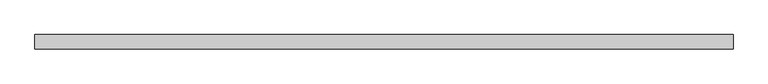
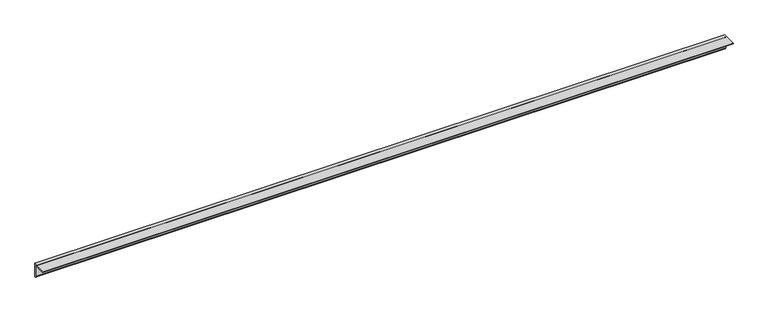
"""IFC4 building model written with IfcOpenShell, lengths in millimetres: member geometry, 0912_Steel Framing_L-KSD3502 : H_SB_AR_S03_L-130x130x12_HBR3."""

from ifc_helpers import new_model, si_unit, point, frame, frame_2d, origin, place, context, project, spatial, polyline, circle_curve, trimmed, segment, composite_curve, outline, extrude, source, transform, mapped, element, save


def member_59aa44e3(model_context):
    return source(origin(), model_context, "Body", "SweptSolid", [
        extrude(outline(composite_curve([segment(polyline([(36.4, 36.4), (36.4, -93.6)]), True, "CONTINUOUS"), segment(trimmed(circle_curve(frame_2d((36.4, -81.6)), 12.0), [point((36.4, -93.6))], [point((24.4, -81.6))], False, "CARTESIAN"), True, "CONTINUOUS"), segment(polyline([(24.4, -81.6), (24.4, 12.4)]), True, "CONTINUOUS"), segment(trimmed(circle_curve(frame_2d((12.4, 12.4)), 12.0), [point((24.4, 12.4))], [point((12.4, 24.4))], True, "CARTESIAN"), True, "CONTINUOUS"), segment(polyline([(12.4, 24.4), (-81.6, 24.4)]), True, "CONTINUOUS"), segment(trimmed(circle_curve(frame_2d((-81.6, 36.4)), 12.0), [point((-81.6, 24.4))], [point((-93.6, 36.4))], False, "CARTESIAN"), True, "CONTINUOUS"), segment(polyline([(-93.6, 36.4), (36.4, 36.4)]), True, "CONTINUOUS")], self_intersect=False)), frame((-3186.8487779, 0.0, 0.0), z_axis=(1.0, 0.0, 0.0), x_axis=(0.0, 1.0, 0.0)), (0.0, 0.0, 1.0), 6284.7404874),
    ])


if __name__ == "__main__":
    model = new_model("IFC4")
    model_context = context("Model", 3, world=origin())
    ifc_project = project(units=[si_unit("LENGTHUNIT", "METRE", prefix="MILLI")], contexts=[model_context])
    site = spatial("IfcSite", under=ifc_project)
    building = spatial("IfcBuilding", under=site)
    placement = place(None, origin())
    member_shape = member_59aa44e3(model_context)
    element("IfcMember", 1, ObjectType="0912_Steel Framing_L-KSD3502 : H_SB_AR_S03_L-130x130x12_HBR3", at=placement, inside=building, context=model_context, shape_type="MappedRepresentation", body=[
        mapped(member_shape, transform((0.0, 0.0, 0.0), x_axis=(1.0, 0.0, 0.0), y_axis=(0.0, 1.0, 0.0), z_axis=(0.0, 0.0, 1.0))),
    ])
    save(model, "model.ifc")

# Revit data of these elements
# Type "0912_Steel Framing_L-KSD3502 : H_SB_AR_S03_L-130x130x12_HBR3"
#   k = 25 mm
#   Perimeter = 0.52 m²/m
#   Nominal Weight = 23.40 kgf/m
#   Length [instance default] = 1000 mm
#   b = 130 mm
#   d = 130 mm
#   t = 12 mm
#   x = 36.4 mm
#   y = 36.4 mm
#   A = 2976.00 m²
#   Structural Material [instance default] = Steel, 45-345
# Element 1 (IfcMember, "0912_Steel Framing_L-KSD3502 : H_SB_AR_S03_L-130x130x12_HBR3")
#   Structural Material = Steel ASTM A36
#   Materials on its faces: "Steel ASTM A36"
# Materials
#   "Steel, 45-345": class "Metal", colour RGB 189 187 185, transparency 0, Description = "Steel 345 MPa", Cost = 0
#   "Steel ASTM A36": class "Metal", colour RGB 199 199 199, transparency 0, Description = "Structural steel, ASTM A36 Grade B, mill finish", Cost = 0
